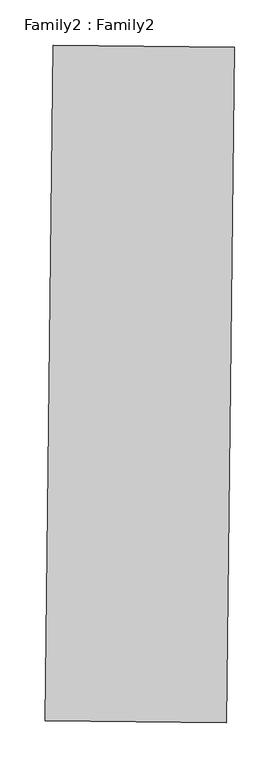
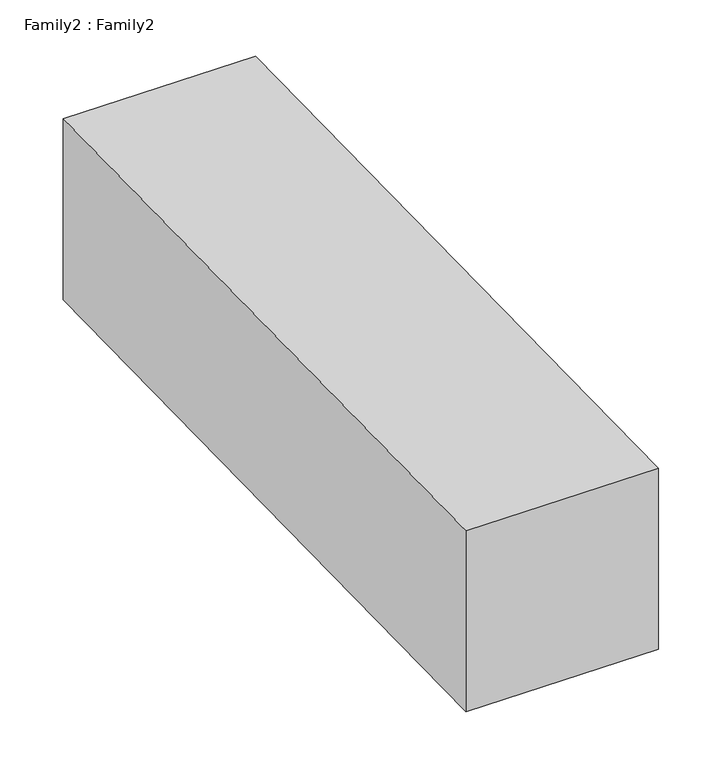
"""IFC4 building model written with IfcOpenShell, lengths in millimetres: proxy geometry, Family2 : Family2."""

from ifc_helpers import new_model, si_unit, origin, place, context, project, spatial, faceted_brep, source, transform, mapped, element, save


def family2_family2_fbbcbc9b(model_context):
    return source(origin(), model_context, "Body", "Brep", [
        faceted_brep([(-3947.7278481, -6445.8117114, 1.0945136), (-3947.7278481, -6445.8117114, 201.0945136), (-3939.1149464, -5701.7884112, 202.060409), (-3939.1149464, -5701.7884112, 2.060409), (-3747.7366581, -6447.6889241, 201.0945136), (-3739.1237564, -5703.6656239, 202.060409), (-3747.7366581, -6447.6889241, 1.0945136), (-3739.1237564, -5703.6656239, 2.060409)], [[[0, 1, 2, 3]], [[1, 4, 5, 2]], [[4, 6, 7, 5]], [[6, 0, 3, 7]], [[3, 2, 5, 7]], [[0, 6, 4, 1]]]),
    ])


if __name__ == "__main__":
    model = new_model("IFC4")
    model_context = context("Model", 3, world=origin())
    ifc_project = project(units=[si_unit("LENGTHUNIT", "METRE", prefix="MILLI")], contexts=[model_context])
    site = spatial("IfcSite", under=ifc_project)
    building = spatial("IfcBuilding", under=site)
    placement = place(None, origin())
    family2_family2_shape = family2_family2_fbbcbc9b(model_context)
    element("IfcBuildingElementProxy", 1, Name="Family2 : Family2", ObjectType="Family2 : Family2", at=placement, inside=building, context=model_context, shape_type="MappedRepresentation", body=[
        mapped(family2_family2_shape, transform((0.0, 0.0, 0.0), x_axis=(1.0, 0.0, 0.0), y_axis=(0.0, 1.0, 0.0), z_axis=(0.0, 0.0, 1.0))),
    ])
    save(model, "model.ifc")

# Revit data of these elements
# Type "Family2 : Family2"
#   Default Elevation = 0
